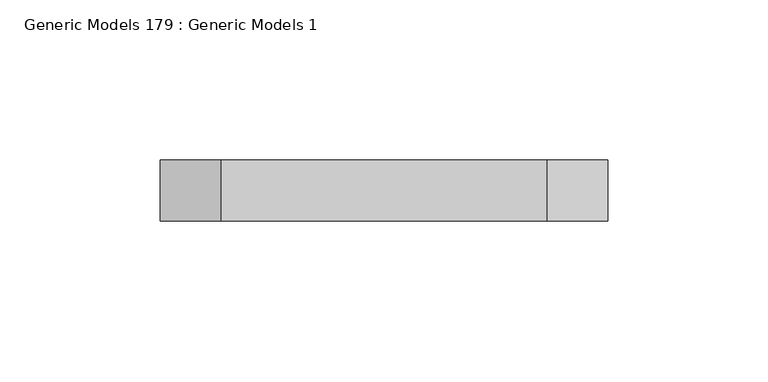
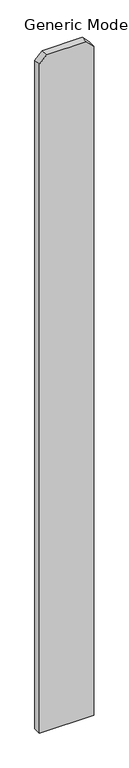
"""IFC4 building model written with IfcOpenShell, lengths in millimetres: proxy geometry, Generic Models 179 : Generic Models 1."""

from ifc_helpers import new_model, si_unit, frame, origin, place, context, project, spatial, polyline, outline, extrude, source, transform, mapped, element, save


def generic_models_179_generic_models_1_da8c2a58(model_context):
    return source(origin(), model_context, "Body", "SweptSolid", [
        extrude(outline(polyline([(76.2, 56970.6125), (1885.95, 56970.6125), (1905.0, 56951.5625), (1905.0, 56849.9625), (1885.95, 56830.9125), (76.2, 56830.9125), (76.2, 56970.6125)])), frame((0.0, 547.6875, 0.0), z_axis=(0.0, 1.0, 0.0), x_axis=(0.0, 0.0, 1.0)), (0.0, 0.0, 1.0), 19.05),
    ])


if __name__ == "__main__":
    model = new_model("IFC4")
    model_context = context("Model", 3, world=origin())
    ifc_project = project(units=[si_unit("LENGTHUNIT", "METRE", prefix="MILLI")], contexts=[model_context])
    site = spatial("IfcSite", under=ifc_project)
    building = spatial("IfcBuilding", under=site)
    placement = place(None, origin())
    generic_models_179_generic_models_1_shape = generic_models_179_generic_models_1_da8c2a58(model_context)
    element("IfcBuildingElementProxy", 1, Name="Generic Models 179 : Generic Models 1", ObjectType="Generic Models 179 : Generic Models 1", at=placement, inside=building, context=model_context, shape_type="MappedRepresentation", body=[
        mapped(generic_models_179_generic_models_1_shape, transform((0.0, 0.0, 0.0), x_axis=(1.0, 0.0, 0.0), y_axis=(0.0, 1.0, 0.0), z_axis=(0.0, 0.0, 1.0))),
    ])
    save(model, "model.ifc")

# Revit data of these elements
# Element 1 (IfcBuildingElementProxy, "Generic Models 179 : Generic Models 1")
#   Materials on its faces: "VERTICAL 1X6 CEDAR PLANKS W/ CLEAR WOOD SEALER"
# Materials
#   "VERTICAL 1X6 CEDAR PLANKS W/ CLEAR WOOD SEALER": class "Wood", colour RGB 234 198 147, transparency 0, Description = "Pinus Echinata", Cost = 0
